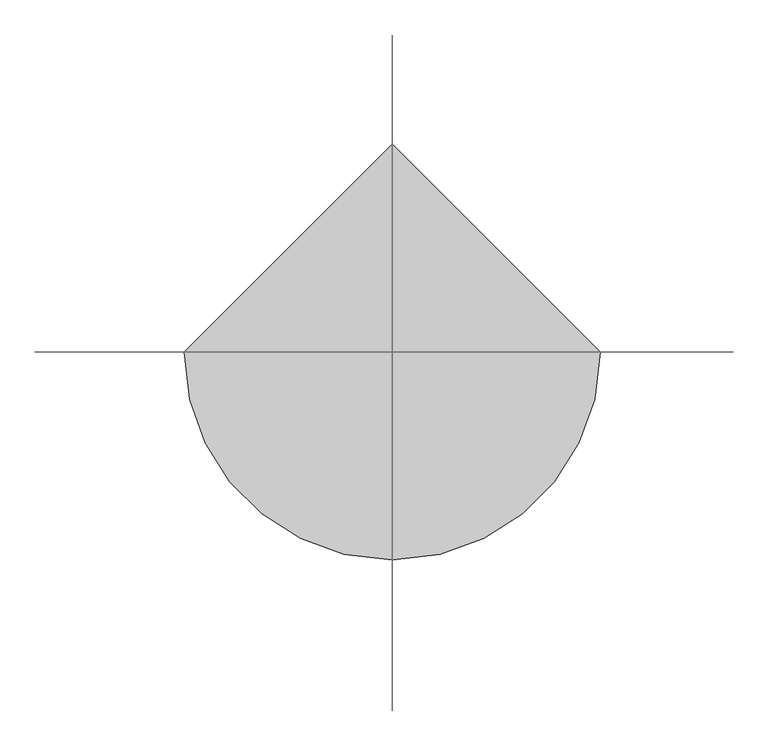
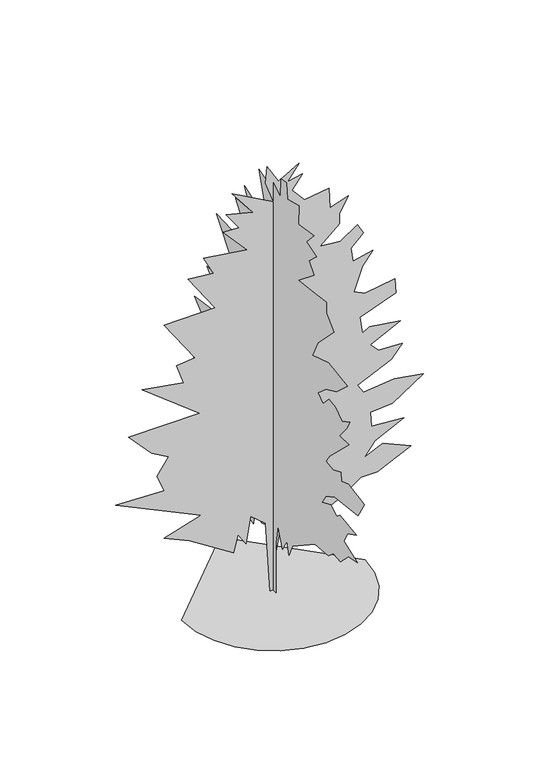
"""IFC4 building model written with IfcOpenShell, lengths in millimetres: proxy geometry, douglas fir 26072 : douglas fir 26072."""

from ifc_helpers import new_model, si_unit, origin, place, context, project, spatial, triangles, source, transform, mapped, element, save


def entourage_30f0a7e8(model_context):
    return source(origin(), model_context, "Body", "Tessellation", [
        triangles([(-1245.1344635, 0.0, 0.000156), (-1212.2185221, -285.3031886, 0.000156), (-1118.4695932, -547.3069273, 0.000156), (-971.3984104, -778.5080767, 0.000156), (-778.5080767, -971.3984104, 0.000156), (-547.3069273, -1118.4695932, 0.000156), (-285.3031886, -1212.2185221, 0.000156), (5.44e-05, -1245.1344635, 0.000156), (285.3031886, -1212.2185221, 0.000156), (547.3069273, -1118.4695932, 0.000156), (778.5080767, -971.3984104, 0.000156), (971.3984104, -778.5080767, 0.000156), (1118.4695932, -547.3069273, 0.000156), (1212.2185221, -285.3031886, 0.000156), (1245.1344635, 0.0001089, 0.000156), (-0.0001633, 1245.1344635, 0.000156), (-42.7741424, 0.0, 0.0), (-102.6564702, -5.92e-05, 994.0450659), (-306.2556524, -6.92e-05, 1161.713102), (-366.1387705, -4.71e-05, 790.44354), (-473.9262683, -5.71e-05, 958.1141922), (-533.8068429, -4.28e-05, 718.5868795), (-1132.6300661, -6.57e-05, 1101.8325274), (-1479.9474564, -7.5e-05, 1257.5245502), (-976.9355724, -8.42e-05, 1413.2189713), (-2138.6512905, -0.0001171, 1964.1353439), (-1479.9474564, -0.0001156, 1940.1830269), (-1575.7589046, -0.0001299, 2179.7104122), (-1420.0643383, -0.0001435, 2407.2641098), (-1647.6155651, -0.0001513, 2539.003743), (-1959.0045525, -0.0001713, 2874.3425766), (-1000.8903603, -0.000172, 2886.3313797), (-1779.3578144, -0.0002084, 3497.1254929), (-1216.4654285, -0.0002027, 3401.316806), (-1312.2768768, -0.0002192, 3676.7546448), (-1060.7708622, -0.0002206, 3700.7066711), (-1479.9474564, -0.000257, 4311.5263641), (-785.3127485, -0.0002577, 4323.4898781), (-1156.5823105, -0.0002898, 4862.4276215), (-809.2649929, -0.0002877, 4826.5117905), (-941.0072422, -0.0003034, 5089.9864059), (-354.1626483, -0.0002984, 5006.1409424), (-677.5252144, -0.0003198, 5365.4492432), (-461.9501824, -0.0003191, 5353.4604401), (-641.5968842, -0.0003341, 5604.9718323), (-270.3273404, -0.0003284, 5509.1625641), (-557.7615944, -0.0003505, 5880.4346695), (5.1314642, -0.0003319, 5569.0304214), (-102.6564702, -0.0003498, 5868.4458664), (-78.70349, -0.0003633, 6096.0046509), (76.9902588, -0.0003476, 5832.5306168), (352.4481454, -0.0003576, 6000.1959641), (196.7543966, -0.0003448, 5784.6259827), (400.3525978, -0.0003476, 5832.5306168), (256.6367334, -0.0003362, 5640.9126617), (424.3073493, -0.0003248, 5449.2697083), (759.6460012, -0.0003277, 5497.173761), (771.6221598, -0.0003105, 5209.7471191), (1023.1280291, -0.0003155, 5293.5925827), (903.3644091, -0.0003034, 5089.9864059), (903.3644091, -0.0002941, 4934.2842819), (639.8823812, -0.0002805, 4706.7507866), (915.3405676, -0.0002791, 4682.7731804), (1142.8917217, -0.0002884, 4838.4753044), (1226.7270115, -0.0002798, 4694.7619835), (1059.0563593, -0.0002698, 4527.0963455), (1083.0111471, -0.0002584, 4335.4786812), (1358.4692608, -0.000262, 4395.3465385), (1214.7509256, -0.0002513, 4215.6920975), (1094.987233, -0.000232, 3892.3499153), (1250.6817993, -0.0002277, 3820.4932549), (1657.8796188, -0.0002313, 3880.3611122), (1669.8557774, -0.0002192, 3676.7546448), (1178.8225954, -0.0002084, 3497.1254929), (1214.7509256, -0.0001942, 3257.5779053), (1310.5623013, -0.0001977, 3317.4713425), (1729.7388954, -0.0001942, 3257.5779053), (1322.5384598, -0.000182, 3053.996727), (1430.3285374, -0.0001749, 2934.2357231), (1753.6910671, -0.0001742, 2922.24692), (1609.9726593, -0.0001635, 2742.5924789), (1142.8917217, -0.0001513, 2539.003743), (1226.7270115, -0.0001435, 2407.2641098), (1645.9036057, -0.0001463, 2455.1684532), (2041.1252666, -0.0001421, 2383.309322), (1621.9488178, -0.0001256, 2107.8511356), (1322.5384598, -0.0001242, 2083.8989639), (1334.514473, -0.0001121, 1880.3000542), (1777.6432388, -0.0001099, 1844.3717239), (1382.4215778, -9.85e-05, 1652.7488274), (1238.70317, -8.78e-05, 1473.1020893), (1490.2090393, -9.42e-05, 1580.8896961), (1873.4546871, -8.42e-05, 1413.2189713), (1418.3497627, -7.14e-05, 1197.6439756), (1190.7986813, -7.14e-05, 1197.6439756), (915.3405676, -6e-05, 1006.0211517), (651.8584671, -5.14e-05, 862.3027439), (520.1187613, -4.43e-05, 742.5391239), (304.5411677, -5.21e-05, 874.2788298), (232.6837442, -4.07e-05, 682.6560059), (112.919343, -5.5e-05, 922.185862), (29.0845483, -2.78e-05, 467.0809739), (41.0606569, 0.0, 0.0), (0.0, 53.1142362, 0.000156), (0.0, 89.0438381, 646.7276756), (0.0, 112.9965639, 850.3266581), (0.0, 268.6890319, 802.4221693), (0.0, 424.3835438, 934.1619478), (0.0, 460.311874, 670.67992), (0.0, 963.3236853, 802.4221693), (0.0, 1574.1204872, 1149.7370161), (0.0, 1166.9226677, 1341.35984), (0.0, 1765.7433838, 1676.7009991), (0.0, 1238.7817989, 1808.4407776), (0.0, 1897.4856331, 2227.6173717), (0.0, 1466.3330257, 2287.5004898), (0.0, 1645.9797638, 2550.9748146), (0.0, 1310.6410755, 2634.8202782), (0.0, 1849.5786736, 3089.912558), (0.0, 1047.1590477, 3209.6735619), (0.0, 1550.1683155, 3700.7066711), (0.0, 1107.0395496, 3724.6589882), (0.0, 1202.8509979, 4048.0267502), (0.0, 939.3715136, 4107.9198967), (0.0, 1334.5932472, 4586.9642029), (0.0, 484.2666255, 4551.0486626), (0.0, 879.4883955, 5089.9864059), (0.0, 532.1710779, 5113.9384323), (0.0, 675.8894857, 5389.4018509), (0.0, 112.9965639, 5197.7838959), (0.0, 184.8552501, 5413.3538773), (0.0, 328.5721318, 5832.5306168), (0.0, 89.0438381, 5760.6739563), (0.0, 124.9729223, 5928.3393036), (0.0, -174.437681, 5748.6851532), (0.0, -186.4143119, 6012.1591873), (0.0, -318.1555801, 6036.111795), (0.0, -342.1077882, 5808.578009), (0.0, -605.589816, 5880.4346695), (0.0, -593.6137301, 5604.9718323), (0.0, -964.8832558, 5664.8646881), (0.0, -785.2365177, 5473.2217346), (0.0, -1024.7638304, 5401.3650742), (0.0, -845.1170923, 5233.6997269), (0.0, -964.8832558, 5101.9496292), (0.0, -593.6137301, 4802.5597641), (0.0, -952.9071699, 4850.4641075), (0.0, -1252.3174553, 4886.3796478), (0.0, -1252.3174553, 4730.7031036), (0.0, -1431.9641933, 4563.0121765), (0.0, -1060.6947041, 4191.7400711), (0.0, -928.9523821, 3928.2654556), (0.0, -1300.221944, 4048.0267502), (0.0, -1755.3268684, 3988.1588928), (0.0, -1491.8448406, 3748.6365944), (0.0, -1240.3414421, 3628.8500107), (0.0, -1060.6947041, 3473.1734665), (0.0, -1168.4822382, 3377.364489), (0.0, -1312.1981026, 3533.0413239), (0.0, -1467.8925236, 3509.0890068), (0.0, -1623.5870899, 3401.316806), (0.0, -1803.233828, 3497.1254929), (0.0, -1731.3745514, 3365.3756859), (0.0, -1563.7039719, 3161.7692184), (0.0, -1779.2790401, 3161.7692184), (0.0, -1324.1767319, 2718.6404526), (0.0, -1240.3414421, 2598.879158), (0.0, -1408.0095509, 2574.9271317), (0.0, -1599.6323021, 2658.7725952), (0.0, -1611.6109314, 2539.003743), (0.0, -1767.3028816, 2586.9159348), (0.0, -2150.5485294, 2527.0277298), (0.0, -1994.8565792, 2275.5217152), (0.0, -1455.9165104, 2215.6412132), (0.0, -1240.3414421, 2095.8751225), (0.0, -1144.5299938, 1952.1591854), (0.0, -1360.1050621, 2047.9706337), (0.0, -1491.8448406, 1964.1353439), (0.0, -1575.6801304, 2024.018462), (0.0, -1958.9257782, 1976.1113571), (0.0, -1755.3268684, 1868.3238956), (0.0, -1671.4915787, 1712.6293293), (0.0, -1982.880566, 1592.8657093), (0.0, -1767.3028816, 1544.9613659), (0.0, -1587.6561436, 1365.3146278), (0.0, -1419.9881802, 1377.290641), (0.0, -1300.221944, 1281.4793381), (0.0, -988.8355001, 1257.5245502), (0.0, -461.8714445, 910.2097034), (0.0, -378.0361184, 730.5630381), (0.0, -330.131666, 898.2336176), (0.0, -222.343387, 718.5868795), (0.0, -114.5556167, 994.0450659), (0.0, -66.6499061, 718.5868795), (0.0, -66.6499061, 0.000156)], [[15, 16, 1], [14, 15, 1], [14, 1, 2], [13, 14, 2], [13, 2, 3], [13, 3, 4], [12, 13, 4], [11, 12, 4], [11, 4, 5], [11, 5, 6], [11, 6, 7], [11, 7, 8], [11, 8, 9], [11, 9, 10], [51, 52, 53], [25, 26, 27], [46, 47, 48], [32, 33, 34], [88, 89, 90], [76, 77, 78], [49, 50, 51], [67, 68, 69], [53, 54, 55], [44, 45, 46], [58, 59, 60], [23, 24, 25], [19, 20, 21], [84, 85, 86], [42, 43, 44], [99, 100, 101], [30, 31, 32], [92, 93, 94], [38, 39, 40], [79, 80, 81], [40, 41, 42], [91, 92, 94], [36, 37, 38], [91, 94, 95], [29, 30, 32], [48, 49, 51], [75, 76, 78], [79, 81, 82], [21, 22, 23], [102, 103, 17], [102, 17, 18], [101, 102, 18], [21, 23, 25], [34, 35, 36], [83, 84, 86], [83, 86, 87], [48, 51, 53], [48, 53, 55], [56, 57, 58], [71, 72, 73], [71, 73, 74], [63, 64, 65], [63, 65, 66], [19, 21, 25], [78, 79, 82], [70, 71, 74], [97, 98, 99], [38, 40, 42], [42, 44, 46], [42, 46, 48], [67, 69, 70], [48, 55, 56], [42, 48, 56], [42, 56, 58], [27, 28, 29], [42, 58, 60], [42, 60, 61], [42, 61, 62], [38, 42, 62], [36, 38, 62], [25, 27, 29], [25, 29, 32], [19, 25, 32], [88, 90, 91], [32, 34, 36], [32, 36, 62], [19, 32, 62], [19, 62, 63], [19, 63, 66], [19, 66, 67], [19, 67, 70], [19, 70, 74], [19, 74, 75], [19, 75, 78], [19, 78, 82], [19, 82, 83], [19, 83, 87], [19, 87, 88], [19, 88, 91], [18, 19, 91], [101, 18, 91], [99, 101, 91], [97, 99, 91], [96, 97, 91], [95, 96, 91], [161, 162, 163], [182, 183, 184], [179, 180, 181], [140, 141, 142], [114, 115, 116], [189, 190, 191], [112, 113, 114], [128, 129, 130], [164, 165, 166], [133, 134, 135], [120, 121, 122], [124, 125, 126], [118, 119, 120], [153, 154, 155], [191, 192, 193], [131, 132, 133], [110, 111, 112], [126, 127, 128], [142, 143, 144], [171, 172, 173], [171, 173, 174], [170, 171, 174], [161, 163, 164], [116, 117, 118], [168, 169, 170], [138, 139, 140], [168, 170, 174], [153, 155, 156], [152, 153, 156], [108, 109, 110], [147, 148, 149], [152, 156, 157], [136, 137, 138], [135, 136, 138], [122, 123, 124], [144, 145, 146], [149, 150, 151], [194, 195, 104], [194, 104, 105], [194, 105, 106], [193, 194, 106], [147, 149, 151], [146, 147, 151], [126, 128, 130], [108, 110, 112], [179, 181, 182], [178, 179, 182], [131, 133, 135], [182, 184, 185], [182, 185, 186], [167, 168, 174], [167, 174, 175], [178, 182, 186], [160, 161, 164], [159, 160, 164], [158, 159, 164], [158, 164, 166], [130, 131, 135], [177, 178, 186], [176, 177, 186], [176, 186, 187], [176, 187, 188], [146, 151, 152], [135, 138, 140], [130, 135, 140], [130, 140, 142], [130, 142, 144], [130, 144, 146], [126, 130, 146], [126, 146, 152], [124, 126, 152], [122, 124, 152], [120, 122, 152], [120, 152, 157], [118, 120, 157], [118, 157, 158], [118, 158, 166], [118, 166, 167], [118, 167, 175], [118, 175, 176], [118, 176, 188], [118, 188, 189], [118, 189, 191], [118, 191, 193], [116, 118, 193], [114, 116, 193], [112, 114, 193], [108, 112, 193], [108, 193, 106], [107, 108, 106]], closed=False),
    ])


if __name__ == "__main__":
    model = new_model("IFC4")
    model_context = context("Model", 3, world=origin())
    ifc_project = project(units=[si_unit("LENGTHUNIT", "METRE", prefix="MILLI")], contexts=[model_context])
    site = spatial("IfcSite", under=ifc_project)
    building = spatial("IfcBuilding", under=site)
    placement = place(None, origin())
    entourage_shape = entourage_30f0a7e8(model_context)
    element("IfcBuildingElementProxy", 1, Name="douglas fir 26072 : douglas fir 26072", ObjectType="douglas fir 26072 : douglas fir 26072", at=placement, inside=building, context=model_context, shape_type="MappedRepresentation", body=[
        mapped(entourage_shape, transform((0.0, 0.0, 0.0), x_axis=(1.0, 0.0, 0.0), y_axis=(0.0, 1.0, 0.0), z_axis=(0.0, 0.0, 1.0))),
    ])
    save(model, "model.ifc")

# Revit data of these elements
# Type "douglas fir 26072 : douglas fir 26072"
#   built-in parameter 1005195 = "RPC-16-FVGW-AKQ0-7N2K-N000-ST1L-LVER-AU"
#   Height = 0
